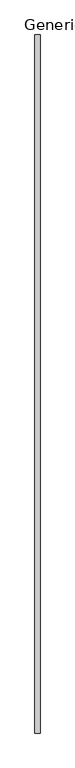
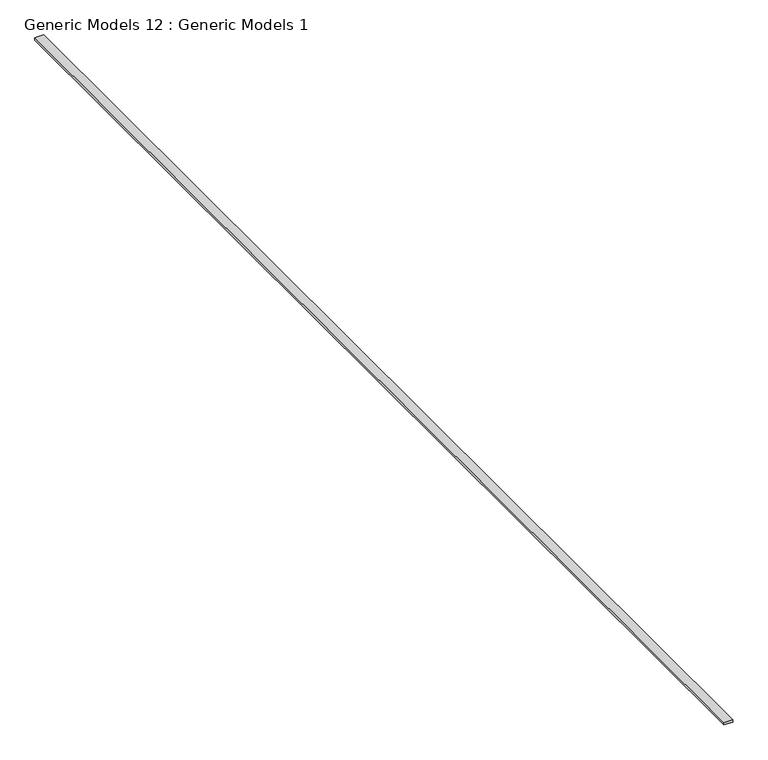
"""IFC4 building model written with IfcOpenShell, lengths in millimetres: proxy geometry, Generic Models 12 : Generic Models 1."""

import ifcopenshell
import ifcopenshell.guid

model = None  # the IFC model being written
_history = None  # IfcOwnerHistory: only IFC2X3 demands one
_inside = {}  # id of a spatial element -> (the spatial element, [elements in it])
_under = {}  # id of a project, library or spatial element -> (it, [spatial elements below it])
_declared = {}  # id of a project -> (the project, [libraries it declares])
_typed = {}  # id of a type object -> (the type object, [elements of that type])
_made_of = {}  # id of a material, layer set ... -> (it, [elements and type objects made of it])


def new_model(schema):
    """Start an empty IFC model of exactly this schema.

    Asked for "IFC4X3", IfcOpenShell would pick the latest addendum, in which some entities
    have other attributes; the version numbers below select the first issue.
    IFC2X3 requires an IfcOwnerHistory on every rooted entity: one is made here for all.
    """
    global model, _history
    if schema == "IFC4X3":
        model = ifcopenshell.file(schema_version=(4, 3, 0, 0))
    else:
        model = ifcopenshell.file(schema=schema)
    _inside.clear()
    _under.clear()
    _declared.clear()
    _typed.clear()
    _made_of.clear()
    _history = None
    if model.schema == "IFC2X3":
        org = make("IfcOrganization", Name="unknown")
        user = make(
            "IfcPersonAndOrganization",
            ThePerson=make("IfcPerson", FamilyName="unknown"),
            TheOrganization=org,
        )
        app = make(
            "IfcApplication",
            ApplicationDeveloper=org,
            Version="unknown",
            ApplicationFullName="unknown",
            ApplicationIdentifier="unknown",
        )
        _history = make(
            "IfcOwnerHistory",
            OwningUser=user,
            OwningApplication=app,
            ChangeAction="ADDED",
            CreationDate=0,
        )
    return model


def make(cls, **values):
    """One entity of the class cls with the attributes given. An attribute that is None is left unset."""
    return model.create_entity(
        cls, **{name: value for name, value in values.items() if value is not None}
    )


def rooted(cls, **values):
    """An entity with a GlobalId (a new one), such as an element, a storey or a relation."""
    return make(cls, GlobalId=ifcopenshell.guid.new(), OwnerHistory=_history, **values)


def si_unit(unit_type, name, prefix=None):
    """IfcSIUnit, for example si_unit("LENGTHUNIT", "METRE", prefix="MILLI")."""
    return make("IfcSIUnit", UnitType=unit_type, Prefix=prefix, Name=name)


def assignment(units):
    """IfcUnitAssignment: the units of a project."""
    return None if units is None else make("IfcUnitAssignment", Units=units)


def point(xyz):
    """IfcCartesianPoint."""
    return None if xyz is None else make("IfcCartesianPoint", Coordinates=xyz)


def direction(xyz):
    """IfcDirection."""
    return None if xyz is None else make("IfcDirection", DirectionRatios=xyz)


def frame(location, z_axis=None, x_axis=None):
    """IfcAxis2Placement3D, a coordinate frame: its origin and axes. An axis left out is left unset."""
    return make(
        "IfcAxis2Placement3D",
        Location=point(location),
        Axis=direction(z_axis),
        RefDirection=direction(x_axis),
    )


def origin():
    """The frame at (0, 0, 0) with its axes left unset."""
    return frame((0.0, 0.0, 0.0))


def place(relative_to, where):
    """IfcLocalPlacement: puts the frame where relative to a parent placement (None: the world)."""
    return make(
        "IfcLocalPlacement", PlacementRelTo=relative_to, RelativePlacement=where
    )


def context(
    kind, dimensions, precision=None, world=None, true_north=None, identifier=None
):
    """IfcGeometricRepresentationContext, for example the 3D "Model" context."""
    return make(
        "IfcGeometricRepresentationContext",
        ContextIdentifier=identifier,
        ContextType=kind,
        CoordinateSpaceDimension=dimensions,
        Precision=precision,
        WorldCoordinateSystem=world,
        TrueNorth=true_north,
    )


def project(units=None, contexts=None):
    """IfcProject with its units and contexts."""
    return rooted(
        "IfcProject",
        Name="project",
        RepresentationContexts=contexts,
        UnitsInContext=assignment(units),
    )


def spatial(cls, under=None, at=None, **own):
    """A site, building, storey or space (cls), placed at a placement, below another one or the project."""
    s = rooted(cls, ObjectPlacement=at, **own)
    if under is not None:
        _under.setdefault(under.id(), (under, []))[1].append(s)
    return s


def polyline(points):
    """IfcPolyline through the points."""
    return make("IfcPolyline", Points=[point(p) for p in points])


def outline(outer, holes=None, kind="AREA"):
    """IfcArbitraryClosedProfileDef: a profile drawn as a closed curve; with holes, ...WithVoids."""
    if holes is None:
        return make("IfcArbitraryClosedProfileDef", ProfileType=kind, OuterCurve=outer)
    return make(
        "IfcArbitraryProfileDefWithVoids",
        ProfileType=kind,
        OuterCurve=outer,
        InnerCurves=holes,
    )


def extrude(swept, where, along, depth):
    """IfcExtrudedAreaSolid: the profile swept, set in the frame where, extruded along a direction by depth."""
    return make(
        "IfcExtrudedAreaSolid",
        SweptArea=swept,
        Position=where,
        ExtrudedDirection=direction(along),
        Depth=depth,
    )


def shape(context_of_items, identifier, shape_type, items):
    """IfcShapeRepresentation: the items that make up one representation, for example the "Body"."""
    return make(
        "IfcShapeRepresentation",
        ContextOfItems=context_of_items,
        RepresentationIdentifier=identifier,
        RepresentationType=shape_type,
        Items=items,
    )


def source(mapping_origin, context_of_items, identifier, shape_type, items):
    """IfcRepresentationMap: a shape defined once, which mapped items show again and again."""
    return make(
        "IfcRepresentationMap",
        MappingOrigin=mapping_origin,
        MappedRepresentation=shape(context_of_items, identifier, shape_type, items),
    )


def transform(
    local_origin,
    x_axis=None,
    y_axis=None,
    z_axis=None,
    scale=None,
    scale2=None,
    scale3=None,
    uniform=True,
):
    """IfcCartesianTransformationOperator3D, or its non-uniform kind. x_axis, y_axis, z_axis: its Axis1, 2, 3."""
    if uniform:
        return make(
            "IfcCartesianTransformationOperator3D",
            Axis1=direction(x_axis),
            Axis2=direction(y_axis),
            LocalOrigin=point(local_origin),
            Scale=scale,
            Axis3=direction(z_axis),
        )
    return make(
        "IfcCartesianTransformationOperator3DnonUniform",
        Axis1=direction(x_axis),
        Axis2=direction(y_axis),
        LocalOrigin=point(local_origin),
        Scale=scale,
        Axis3=direction(z_axis),
        Scale2=scale2,
        Scale3=scale3,
    )


def mapped(mapping_source, mapping_target):
    """IfcMappedItem: shows the shape of a source again, moved by a transform."""
    return make(
        "IfcMappedItem", MappingSource=mapping_source, MappingTarget=mapping_target
    )


def made_of(thing, what):
    """Note that an element or type object is made of a material, layer set ...; save() writes the relation."""
    if what is not None:
        _made_of.setdefault(what.id(), (what, []))[1].append(thing)
    return thing


def element(
    cls,
    number,
    at=None,
    inside=None,
    cuts=None,
    type_object=None,
    material=None,
    context=None,
    identifier="Body",
    shape_type=None,
    held_by="IfcProductDefinitionShape",
    body=None,
    shapes=None,
    **own,
):
    """One element of the class cls, such as IfcWall. Its Tag is "e" and its number.

    at: its placement. inside: the storey or other place that contains it. cuts: it is an
    opening in that element (IfcRelVoidsElement). A single representation is given by context,
    identifier, shape_type and body (its items); several are given by shapes. held_by: the class
    of the entity that holds the representations. save() writes the other relations.
    """
    e = rooted(cls, Tag="e%d" % number, ObjectPlacement=at, **own)
    if body is not None:
        shapes = [shape(context, identifier, shape_type, body)]
    if shapes is not None:
        e.Representation = make(held_by, Representations=shapes)
    if inside is not None:
        _inside.setdefault(inside.id(), (inside, []))[1].append(e)
    if cuts is not None:
        rooted(
            "IfcRelVoidsElement", RelatingBuildingElement=cuts, RelatedOpeningElement=e
        )
    if type_object is not None:
        _typed.setdefault(type_object.id(), (type_object, []))[1].append(e)
    return made_of(e, material)


def aggregate(whole, parts):
    """IfcRelAggregates: a whole, such as a stair, and the parts it consists of."""
    return rooted("IfcRelAggregates", RelatingObject=whole, RelatedObjects=parts)


def save(model, path):
    """Write the relations noted so far, then the file.

    IfcRelAggregates (storeys below a building ...), IfcRelContainedInSpatialStructure (elements
    in a storey), IfcRelDefinesByType, IfcRelAssociatesMaterial and IfcRelDeclares: one each for
    every whole, place, type object, material and project.
    """
    for whole, parts in _under.values():
        aggregate(whole, parts)
    for where, things in _inside.values():
        rooted(
            "IfcRelContainedInSpatialStructure",
            RelatedElements=things,
            RelatingStructure=where,
        )
    for kind, things in _typed.values():
        rooted("IfcRelDefinesByType", RelatedObjects=things, RelatingType=kind)
    for what, things in _made_of.values():
        rooted("IfcRelAssociatesMaterial", RelatedObjects=things, RelatingMaterial=what)
    for by, libraries in _declared.values():
        rooted("IfcRelDeclares", RelatingContext=by, RelatedDefinitions=libraries)
    model.write(path)


def generic_models_12_generic_models_1_ed9a0c98(model_context):
    return source(origin(), model_context, "Body", "SweptSolid", [
        extrude(outline(polyline([(8435.8013705, 11981.8769662), (8575.5013705, 11981.8769662), (8575.5013705, -7068.1230338), (8435.8013705, -7068.1230338), (8435.8013705, 11981.8769662)])), frame((0.0, 0.0, 127028.2735933), z_axis=(0.0, 0.0, 1.0), x_axis=(1.0, 0.0, 0.0)), (0.0, 0.0, 1.0), 38.1),
    ])


if __name__ == "__main__":
    model = new_model("IFC4")
    model_context = context("Model", 3, world=origin())
    ifc_project = project(units=[si_unit("LENGTHUNIT", "METRE", prefix="MILLI")], contexts=[model_context])
    site = spatial("IfcSite", under=ifc_project)
    building = spatial("IfcBuilding", under=site)
    placement = place(None, origin())
    generic_models_12_generic_models_1_shape = generic_models_12_generic_models_1_ed9a0c98(model_context)
    element("IfcBuildingElementProxy", 1, Name="Generic Models 12 : Generic Models 1", ObjectType="Generic Models 12 : Generic Models 1", at=placement, inside=building, context=model_context, shape_type="MappedRepresentation", body=[
        mapped(generic_models_12_generic_models_1_shape, transform((0.0, 0.0, 0.0), x_axis=(1.0, 0.0, 0.0), y_axis=(0.0, 1.0, 0.0), z_axis=(0.0, 0.0, 1.0))),
    ])
    save(model, "model.ifc")

# Revit data of these elements
# Element 1 (IfcBuildingElementProxy, "Generic Models 12 : Generic Models 1")
#   Materials on its faces: "_2X BLOCKING AS REQUIRED"
# Materials
#   "_2X BLOCKING AS REQUIRED": class "Generic", colour RGB 177 130 114, transparency 0, Cost = 0
